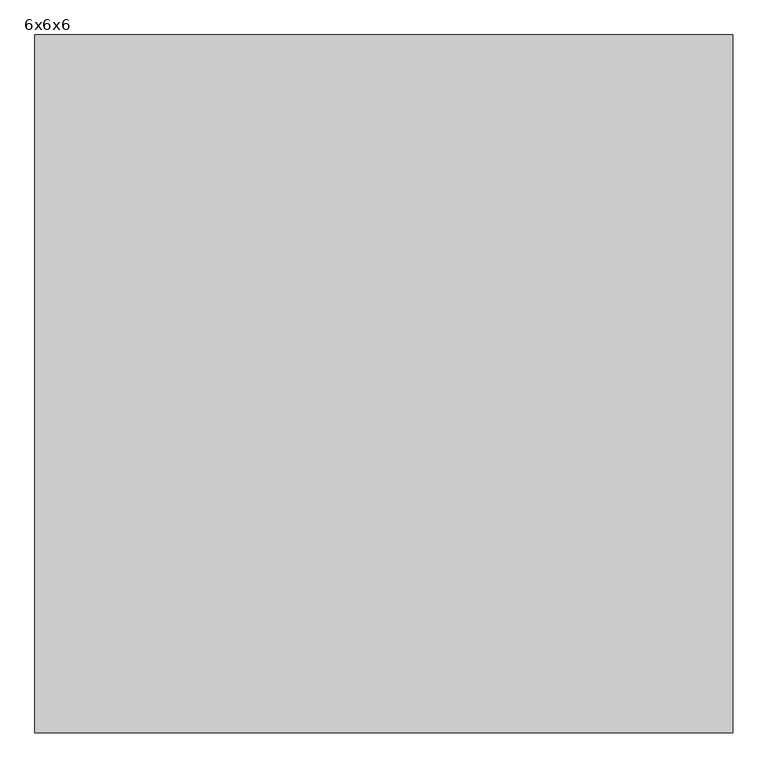
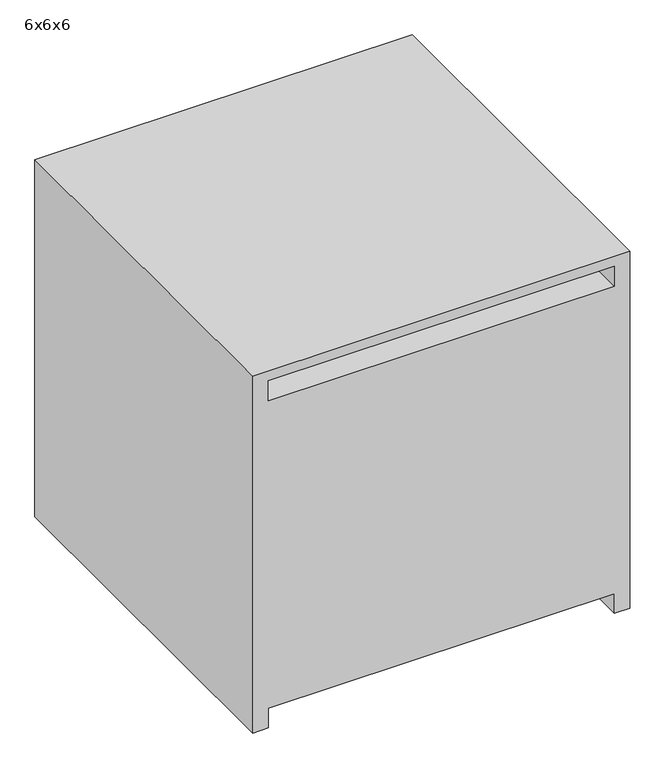
"""IFC4 building model written with IfcOpenShell, lengths in millimetres: proxy geometry, Transformer-Dry-Type-Siemens : 6x6x6."""

from ifc_helpers import new_model, si_unit, frame, origin, place, context, project, spatial, polyline, outline, extrude, source, transform, mapped, element, save


def proxy_6x6x6_c494abd1(model_context):
    return source(origin(), model_context, "Body", "SweptSolid", [
        extrude(outline(polyline([(1828.8, 914.4), (1828.8, -914.4), (0.0, -914.4), (0.0, -838.2), (101.6, -838.2), (101.6, 838.2), (0.0, 838.2), (0.0, 914.4), (1828.8, 914.4)]), holes=[polyline([(1778.0, 838.2), (1676.4, 838.2), (1676.4, -838.2), (1778.0, -838.2), (1778.0, 838.2)])]), frame((0.0, -914.4, 0.0), z_axis=(0.0, 1.0, 0.0), x_axis=(0.0, 0.0, 1.0)), (0.0, 0.0, 1.0), 1828.8),
    ])


if __name__ == "__main__":
    model = new_model("IFC4")
    model_context = context("Model", 3, world=origin())
    ifc_project = project(units=[si_unit("LENGTHUNIT", "METRE", prefix="MILLI")], contexts=[model_context])
    site = spatial("IfcSite", under=ifc_project)
    building = spatial("IfcBuilding", under=site)
    placement = place(None, origin())
    proxy_6x6x6_shape = proxy_6x6x6_c494abd1(model_context)
    element("IfcBuildingElementProxy", 1, Name="Transformer-Dry-Type-Siemens : 6x6x6", ObjectType="Transformer-Dry-Type-Siemens : 6x6x6", at=placement, inside=building, context=model_context, shape_type="MappedRepresentation", body=[
        mapped(proxy_6x6x6_shape, transform((0.0, 0.0, 0.0), x_axis=(1.0, 0.0, 0.0), y_axis=(0.0, 1.0, 0.0), z_axis=(0.0, 0.0, 1.0))),
    ])
    save(model, "model.ifc")

# Revit data of these elements
# Type "Transformer-Dry-Type-Siemens : 6x6x6"
#   Weight = "5500"
#   Wattage = "DO NOT USE"
#   Voltage = "DO NOT USE"
#   URL = "http://www.usa.siemens.com/ce"
#   Transformer Material = "Aluminum"
#   Product Page URL = "http://www.sea.siemens.com/us/Products/PowerDistribution/Product/Transformers/Pages/Transformers.aspx"
#   Product Documentation Link = "http://www.sea.siemens.com/us/internet-dms/Internet/ConsultingEngineersComm/General/Docs/drytrans.pdf"
#   Model = "3F3Y015K13TP1"
#   Manufacturer = "Siemens Industry"
#   KVA = "750"
#   K Factor = "13"
#   Description = "Transformer"
#   Deg Rise = "150"
#   Copyright © = "© Siemens Industry, Inc. 2011"
#   CTRL Connector Description = "Equipment Power"
#   BOM URL [instance default] = ""
#   Assembly Code = "D5090900"
#   clearance = 3' - 0"
#   Width = 6' - 0"
#   Primary Voltage = 480 V
#   Power Factor = 1
#   Height = 6' - 0"
#   Depth = 6' - 0"
#   Apparent Load [instance default] = 0 VA
#   Has Not Contacted Siemens For Configuration [instance default] = no
#   Contacted Siemens For Configuration [instance default] = yes
#   Text Material = Paint- Siemens - Dark
#   Frame Material = Metal - Siemens - Steel
# Element 1 (IfcBuildingElementProxy, "Transformer-Dry-Type-Siemens : 6x6x6")
#   Materials on its faces: "Metal - Siemens - Steel"
# Materials
#   "Paint- Siemens - Dark": class "Metal", colour RGB 175 38 68, transparency 0
#   "Metal - Siemens - Steel": class "Metal", colour RGB 63 114 97, transparency 0, Cost = 0
